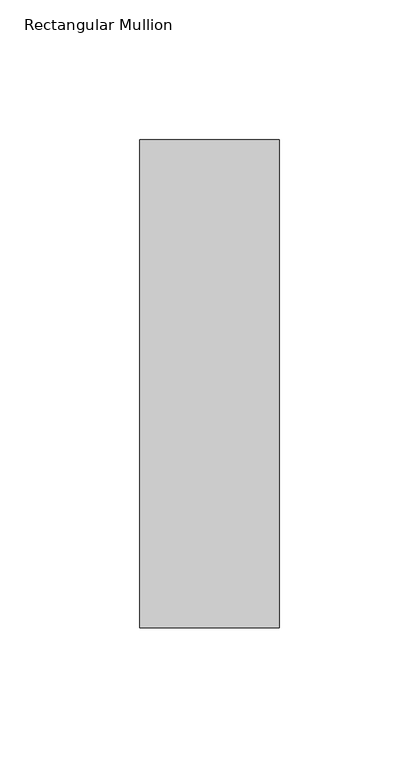
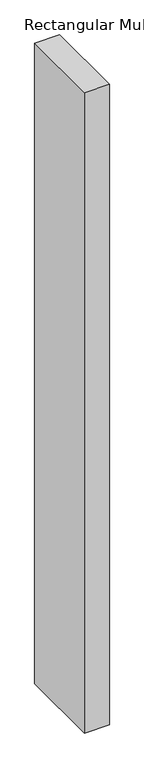
"""IFC4 building model written with IfcOpenShell, lengths in millimetres: member geometry, Rectangular Mullion : WWm-50x175-50mmOffset."""

from ifc_helpers import new_model, si_unit, frame, origin, place, context, project, spatial, polyline, outline, extrude, source, transform, mapped, element, save


def rectangular_mullion_5fcd120d(model_context):
    return source(origin(), model_context, "Body", "SweptSolid", [
        extrude(outline(polyline([(0.0, 87.5), (0.0, -87.5), (-50.0, -87.5), (-50.0, 87.5), (0.0, 87.5)])), frame((0.0, 0.0, -1370.6611397), z_axis=(0.0, 0.0, 1.0), x_axis=(1.0, 0.0, 0.0)), (0.0, 0.0, 1.0), 1370.6611397),
    ])


if __name__ == "__main__":
    model = new_model("IFC4")
    model_context = context("Model", 3, world=origin())
    ifc_project = project(units=[si_unit("LENGTHUNIT", "METRE", prefix="MILLI")], contexts=[model_context])
    site = spatial("IfcSite", under=ifc_project)
    building = spatial("IfcBuilding", under=site)
    placement = place(None, origin())
    rectangular_mullion_shape = rectangular_mullion_5fcd120d(model_context)
    element("IfcMember", 1, ObjectType="Rectangular Mullion : WWm-50x175-50mmOffset", at=placement, inside=building, context=model_context, shape_type="MappedRepresentation", body=[
        mapped(rectangular_mullion_shape, transform((0.0, 0.0, 0.0), x_axis=(1.0, 0.0, 0.0), y_axis=(0.0, 1.0, 0.0), z_axis=(0.0, 0.0, 1.0))),
    ])
    save(model, "model.ifc")

# Revit data of these elements
# Type "Rectangular Mullion : WWm-50x175-50mmOffset"
#   built-in parameter 1007304 = 0.574147 (stored number, unit not read)
#   built-in parameter 1007301 = 0.082021 (stored number, unit not read)
#   built-in parameter 1007300 = 0.082021 (stored number, unit not read)
# Element 1 (IfcMember, "Rectangular Mullion : WWm-50x175-50mmOffset")
#   Materials on its faces: "WW-EC-RGB-Mullion"
# Materials
#   "WW-EC-RGB-Mullion": class "Generic", colour RGB 255 255 255, transparency 0, Comments = "If region requests black mullions, switch asset color to RGB 25-25-25", Description = "Generic Color", Cost = 0
